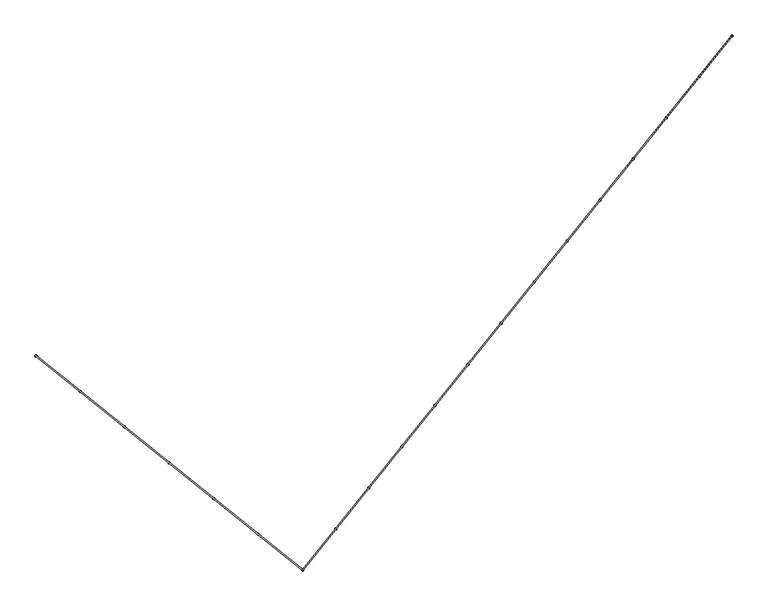
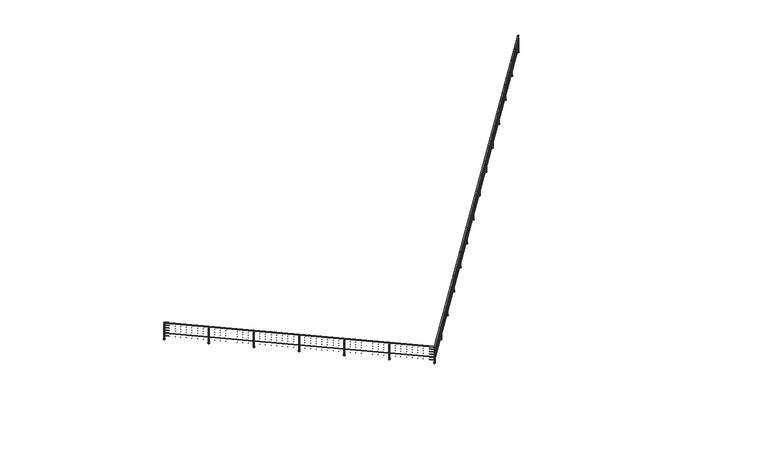
"""IFC4 building model written with IfcOpenShell, lengths in millimetres: railing geometry."""

from ifc_helpers import new_model, si_unit, point, frame, frame_2d, origin, place, context, project, spatial, circle_curve, ellipse_curve, trimmed, segment, composite_curve, outline, extrude, source, transform, mapped, element, save
from ifc_brep_helpers import plane_surface, cylinder_surface, advanced_brep


def railing_283a873e(model_context):
    return source(origin(), model_context, "Body", "SolidModel", [
        advanced_brep(
        [(16703.9390203, 14071.9773332, 12197.5), (16700.0406554, 14075.1082677, 12197.5), (-9274.6280116, 2130.9946489, 12197.5), (-9271.4970771, 2134.8930138, 12197.5), (687.6435705, -5870.1084734, 12197.5), (686.8761401, -5863.0791739, 12197.5)],
        [
            (0, 1, circle_curve(frame((16701.9898378, 14073.5428004, 12197.5), z_axis=(0.6261869005875139, 0.7796729862786083, 0.0), x_axis=(-0.7796729862786083, 0.6261869005875139, 0.0)), 2.5)),
            (1, 0, circle_curve(frame((16701.9898378, 14073.5428004, 12197.5), z_axis=(0.6261869005875139, 0.7796729862786083, 0.0), x_axis=(-0.7796729862786083, 0.6261869005875139, 0.0)), 2.5)),
            (2, 3, circle_curve(frame((-9273.0625444, 2132.9438313, 12197.5), z_axis=(-0.7796729862786094, 0.6261869005875127, 0.0), x_axis=(0.6261869005875127, 0.7796729862786094, 0.0)), 2.5)),
            (3, 2, circle_curve(frame((-9273.0625444, 2132.9438313, 12197.5), z_axis=(-0.7796729862786094, 0.6261869005875127, 0.0), x_axis=(0.6261869005875127, 0.7796729862786094, 0.0)), 2.5)),
            (0, 4),
            (4, 5, ellipse_curve(frame((687.2598553, -5866.5938237, 12197.5), z_axis=(0.9940930594011873, 0.1085310520099531, 0.0), x_axis=(-0.10853105200995282, 0.9940930594011875, 0.0)), 3.5355339, 2.5)),
            (5, 1),
            (5, 4, ellipse_curve(frame((687.2598553, -5866.5938237, 12197.5), z_axis=(0.9940930594011873, 0.1085310520099531, 0.0), x_axis=(-0.10853105200995282, 0.9940930594011875, 0.0)), 3.5355339, 2.5)),
            (4, 2),
            (3, 5),
        ],
        [
            plane_surface(frame((16701.9898378, 14073.5428004, 12200.0), z_axis=(0.6261869005875139, 0.7796729862786083, 0.0), x_axis=(0.7796729862786083, -0.6261869005875139, 0.0))),
            plane_surface(frame((-9273.0625444, 2132.9438313, 12200.0), z_axis=(-0.7796729862786096, 0.6261869005875125, 0.0), x_axis=(0.6261869005875125, 0.7796729862786096, 0.0))),
            cylinder_surface(frame((16701.9898378, 14073.5428004, 12197.5), z_axis=(0.6261869005875139, 0.7796729862786083, 0.0), x_axis=(-0.7796729862786083, 0.6261869005875139, 0.0)), 2.5),
            cylinder_surface(frame((687.2598553, -5866.5938237, 12197.5), z_axis=(0.7796729862786094, -0.6261869005875127, 0.0), x_axis=(0.6261869005875127, 0.7796729862786094, 0.0)), 2.5),
        ],
        [
            (0, [[1, 2]]),
            (1, [[3, 4]]),
            (2, [[-1, 5, 6, 7]]),
            (2, [[-2, -7, 8, -5]]),
            (3, [[-6, 9, -4, 10]]),
            (3, [[-8, -10, -3, -9]]),
        ],
    ),
        advanced_brep(
        [(16703.9390203, 14071.9773332, 12347.5), (16700.0406554, 14075.1082677, 12347.5), (-9274.6280116, 2130.9946489, 12347.5), (-9271.4970771, 2134.8930138, 12347.5), (687.6435705, -5870.1084734, 12347.5), (686.8761401, -5863.0791739, 12347.5)],
        [
            (0, 1, circle_curve(frame((16701.9898378, 14073.5428004, 12347.5), z_axis=(0.6261869005875139, 0.7796729862786083, 0.0), x_axis=(-0.7796729862786083, 0.6261869005875139, 0.0)), 2.5)),
            (1, 0, circle_curve(frame((16701.9898378, 14073.5428004, 12347.5), z_axis=(0.6261869005875139, 0.7796729862786083, 0.0), x_axis=(-0.7796729862786083, 0.6261869005875139, 0.0)), 2.5)),
            (2, 3, circle_curve(frame((-9273.0625444, 2132.9438313, 12347.5), z_axis=(-0.7796729862786094, 0.6261869005875127, 0.0), x_axis=(0.6261869005875127, 0.7796729862786094, 0.0)), 2.5)),
            (3, 2, circle_curve(frame((-9273.0625444, 2132.9438313, 12347.5), z_axis=(-0.7796729862786094, 0.6261869005875127, 0.0), x_axis=(0.6261869005875127, 0.7796729862786094, 0.0)), 2.5)),
            (0, 4),
            (4, 5, ellipse_curve(frame((687.2598553, -5866.5938237, 12347.5), z_axis=(0.9940930594011873, 0.1085310520099531, 0.0), x_axis=(-0.10853105200995282, 0.9940930594011875, 0.0)), 3.5355339, 2.5)),
            (5, 1),
            (5, 4, ellipse_curve(frame((687.2598553, -5866.5938237, 12347.5), z_axis=(0.9940930594011873, 0.1085310520099531, 0.0), x_axis=(-0.10853105200995282, 0.9940930594011875, 0.0)), 3.5355339, 2.5)),
            (4, 2),
            (3, 5),
        ],
        [
            plane_surface(frame((16701.9898378, 14073.5428004, 12350.0), z_axis=(0.6261869005875139, 0.7796729862786083, 0.0), x_axis=(0.7796729862786083, -0.6261869005875139, 0.0))),
            plane_surface(frame((-9273.0625444, 2132.9438313, 12350.0), z_axis=(-0.7796729862786096, 0.6261869005875125, 0.0), x_axis=(0.6261869005875125, 0.7796729862786096, 0.0))),
            cylinder_surface(frame((16701.9898378, 14073.5428004, 12347.5), z_axis=(0.6261869005875139, 0.7796729862786083, 0.0), x_axis=(-0.7796729862786083, 0.6261869005875139, 0.0)), 2.5),
            cylinder_surface(frame((687.2598553, -5866.5938237, 12347.5), z_axis=(0.7796729862786094, -0.6261869005875127, 0.0), x_axis=(0.6261869005875127, 0.7796729862786094, 0.0)), 2.5),
        ],
        [
            (0, [[1, 2]]),
            (1, [[3, 4]]),
            (2, [[-1, 5, 6, 7]]),
            (2, [[-2, -7, 8, -5]]),
            (3, [[-6, 9, -4, 10]]),
            (3, [[-8, -10, -3, -9]]),
        ],
    ),
        advanced_brep(
        [(16703.9390203, 14071.9773332, 12497.5), (16700.0406554, 14075.1082677, 12497.5), (-9274.6280116, 2130.9946489, 12497.5), (-9271.4970771, 2134.8930138, 12497.5), (687.6435705, -5870.1084734, 12497.5), (686.8761401, -5863.0791739, 12497.5)],
        [
            (0, 1, circle_curve(frame((16701.9898378, 14073.5428004, 12497.5), z_axis=(0.6261869005875139, 0.7796729862786083, 0.0), x_axis=(-0.7796729862786083, 0.6261869005875139, 0.0)), 2.5)),
            (1, 0, circle_curve(frame((16701.9898378, 14073.5428004, 12497.5), z_axis=(0.6261869005875139, 0.7796729862786083, 0.0), x_axis=(-0.7796729862786083, 0.6261869005875139, 0.0)), 2.5)),
            (2, 3, circle_curve(frame((-9273.0625444, 2132.9438313, 12497.5), z_axis=(-0.7796729862786094, 0.6261869005875127, 0.0), x_axis=(0.6261869005875127, 0.7796729862786094, 0.0)), 2.5)),
            (3, 2, circle_curve(frame((-9273.0625444, 2132.9438313, 12497.5), z_axis=(-0.7796729862786094, 0.6261869005875127, 0.0), x_axis=(0.6261869005875127, 0.7796729862786094, 0.0)), 2.5)),
            (0, 4),
            (4, 5, ellipse_curve(frame((687.2598553, -5866.5938237, 12497.5), z_axis=(0.9940930594011873, 0.1085310520099531, 0.0), x_axis=(-0.10853105200995282, 0.9940930594011875, 0.0)), 3.5355339, 2.5)),
            (5, 1),
            (5, 4, ellipse_curve(frame((687.2598553, -5866.5938237, 12497.5), z_axis=(0.9940930594011873, 0.1085310520099531, 0.0), x_axis=(-0.10853105200995282, 0.9940930594011875, 0.0)), 3.5355339, 2.5)),
            (4, 2),
            (3, 5),
        ],
        [
            plane_surface(frame((16701.9898378, 14073.5428004, 12500.0), z_axis=(0.6261869005875139, 0.7796729862786083, 0.0), x_axis=(0.7796729862786083, -0.6261869005875139, 0.0))),
            plane_surface(frame((-9273.0625444, 2132.9438313, 12500.0), z_axis=(-0.7796729862786096, 0.6261869005875125, 0.0), x_axis=(0.6261869005875125, 0.7796729862786096, 0.0))),
            cylinder_surface(frame((16701.9898378, 14073.5428004, 12497.5), z_axis=(0.6261869005875139, 0.7796729862786083, 0.0), x_axis=(-0.7796729862786083, 0.6261869005875139, 0.0)), 2.5),
            cylinder_surface(frame((687.2598553, -5866.5938237, 12497.5), z_axis=(0.7796729862786094, -0.6261869005875127, 0.0), x_axis=(0.6261869005875127, 0.7796729862786094, 0.0)), 2.5),
        ],
        [
            (0, [[1, 2]]),
            (1, [[3, 4]]),
            (2, [[-1, 5, 6, 7]]),
            (2, [[-2, -7, 8, -5]]),
            (3, [[-6, 9, -4, 10]]),
            (3, [[-8, -10, -3, -9]]),
        ],
    ),
        advanced_brep(
        [(16703.9390203, 14071.9773332, 12647.5), (16700.0406554, 14075.1082677, 12647.5), (687.6435705, -5870.1084734, 12647.5), (686.8761401, -5863.0791739, 12647.5), (-9274.6280116, 2130.9946489, 12647.5), (-9271.4970771, 2134.8930138, 12647.5)],
        [
            (0, 1, circle_curve(frame((16701.9898378, 14073.5428004, 12647.5), z_axis=(0.6261869005875139, 0.7796729862786083, 0.0), x_axis=(-0.7796729862786083, 0.6261869005875139, 0.0)), 2.5)),
            (1, 0, circle_curve(frame((16701.9898378, 14073.5428004, 12647.5), z_axis=(0.6261869005875139, 0.7796729862786083, 0.0), x_axis=(-0.7796729862786083, 0.6261869005875139, 0.0)), 2.5)),
            (0, 2),
            (2, 3, ellipse_curve(frame((687.2598553, -5866.5938237, 12647.5), z_axis=(0.9940930594011873, 0.1085310520099531, 0.0), x_axis=(-0.10853105200995282, 0.9940930594011875, 0.0)), 3.5355339, 2.5)),
            (3, 1),
            (3, 2, ellipse_curve(frame((687.2598553, -5866.5938237, 12647.5), z_axis=(0.9940930594011873, 0.1085310520099531, 0.0), x_axis=(-0.10853105200995282, 0.9940930594011875, 0.0)), 3.5355339, 2.5)),
            (4, 5, circle_curve(frame((-9273.0625444, 2132.9438313, 12647.5), z_axis=(-0.7796729862786094, 0.6261869005875127, 0.0), x_axis=(0.6261869005875127, 0.7796729862786094, 0.0)), 2.5)),
            (5, 4, circle_curve(frame((-9273.0625444, 2132.9438313, 12647.5), z_axis=(-0.7796729862786094, 0.6261869005875127, 0.0), x_axis=(0.6261869005875127, 0.7796729862786094, 0.0)), 2.5)),
            (2, 4),
            (5, 3),
        ],
        [
            plane_surface(frame((16701.9898378, 14073.5428004, 12650.0), z_axis=(0.6261869005875139, 0.7796729862786083, 0.0), x_axis=(0.7796729862786083, -0.6261869005875139, 0.0))),
            cylinder_surface(frame((16701.9898378, 14073.5428004, 12647.5), z_axis=(0.6261869005875139, 0.7796729862786083, 0.0), x_axis=(-0.7796729862786083, 0.6261869005875139, 0.0)), 2.5),
            plane_surface(frame((-9273.0625444, 2132.9438313, 12650.0), z_axis=(-0.7796729862786096, 0.6261869005875125, 0.0), x_axis=(0.6261869005875125, 0.7796729862786096, 0.0))),
            cylinder_surface(frame((687.2598553, -5866.5938237, 12647.5), z_axis=(0.7796729862786094, -0.6261869005875127, 0.0), x_axis=(0.6261869005875127, 0.7796729862786094, 0.0)), 2.5),
        ],
        [
            (0, [[1, 2]]),
            (1, [[-1, 3, 4, 5]]),
            (1, [[-2, -5, 6, -3]]),
            (2, [[7, 8]]),
            (3, [[-4, 9, -8, 10]]),
            (3, [[-6, -10, -7, -9]]),
        ],
    ),
        advanced_brep(
        [(16703.9390203, 14071.9773332, 12797.5), (16700.0406554, 14075.1082677, 12797.5), (687.6435705, -5870.1084734, 12797.5), (686.8761401, -5863.0791739, 12797.5), (-9274.6280116, 2130.9946489, 12797.5), (-9271.4970771, 2134.8930138, 12797.5)],
        [
            (0, 1, circle_curve(frame((16701.9898378, 14073.5428004, 12797.5), z_axis=(0.6261869005875139, 0.7796729862786083, 0.0), x_axis=(-0.7796729862786083, 0.6261869005875139, 0.0)), 2.5)),
            (1, 0, circle_curve(frame((16701.9898378, 14073.5428004, 12797.5), z_axis=(0.6261869005875139, 0.7796729862786083, 0.0), x_axis=(-0.7796729862786083, 0.6261869005875139, 0.0)), 2.5)),
            (0, 2),
            (2, 3, ellipse_curve(frame((687.2598553, -5866.5938237, 12797.5), z_axis=(0.9940930594011873, 0.1085310520099531, 0.0), x_axis=(-0.10853105200995282, 0.9940930594011875, 0.0)), 3.5355339, 2.5)),
            (3, 1),
            (3, 2, ellipse_curve(frame((687.2598553, -5866.5938237, 12797.5), z_axis=(0.9940930594011873, 0.1085310520099531, 0.0), x_axis=(-0.10853105200995282, 0.9940930594011875, 0.0)), 3.5355339, 2.5)),
            (4, 5, circle_curve(frame((-9273.0625444, 2132.9438313, 12797.5), z_axis=(-0.7796729862786094, 0.6261869005875127, 0.0), x_axis=(0.6261869005875127, 0.7796729862786094, 0.0)), 2.5)),
            (5, 4, circle_curve(frame((-9273.0625444, 2132.9438313, 12797.5), z_axis=(-0.7796729862786094, 0.6261869005875127, 0.0), x_axis=(0.6261869005875127, 0.7796729862786094, 0.0)), 2.5)),
            (2, 4),
            (5, 3),
        ],
        [
            plane_surface(frame((16701.9898378, 14073.5428004, 12800.0), z_axis=(0.6261869005875139, 0.7796729862786083, 0.0), x_axis=(0.7796729862786083, -0.6261869005875139, 0.0))),
            cylinder_surface(frame((16701.9898378, 14073.5428004, 12797.5), z_axis=(0.6261869005875139, 0.7796729862786083, 0.0), x_axis=(-0.7796729862786083, 0.6261869005875139, 0.0)), 2.5),
            plane_surface(frame((-9273.0625444, 2132.9438313, 12800.0), z_axis=(-0.7796729862786096, 0.6261869005875125, 0.0), x_axis=(0.6261869005875125, 0.7796729862786096, 0.0))),
            cylinder_surface(frame((687.2598553, -5866.5938237, 12797.5), z_axis=(0.7796729862786094, -0.6261869005875127, 0.0), x_axis=(0.6261869005875127, 0.7796729862786094, 0.0)), 2.5),
        ],
        [
            (0, [[1, 2]]),
            (1, [[-1, 3, 4, 5]]),
            (1, [[-2, -5, 6, -3]]),
            (2, [[7, 8]]),
            (3, [[-4, 9, -8, 10]]),
            (3, [[-6, -10, -7, -9]]),
        ],
    ),
        advanced_brep(
        [(16721.4816625, 14057.8881279, 12925.0), (16682.4980132, 14089.1974729, 12925.0), (691.0970075, -5901.7403208, 12925.0), (683.4227032, -5831.4473265, 12925.0), (-9288.7172169, 2113.4520067, 12925.0), (-9257.4078719, 2152.435656, 12925.0)],
        [
            (0, 1, circle_curve(frame((16701.9898378, 14073.5428004, 12925.0), z_axis=(0.6261869005875139, 0.7796729862786083, 0.0), x_axis=(-0.7796729862786083, 0.6261869005875139, 0.0)), 25.0)),
            (1, 0, circle_curve(frame((16701.9898378, 14073.5428004, 12925.0), z_axis=(0.6261869005875139, 0.7796729862786083, 0.0), x_axis=(-0.7796729862786083, 0.6261869005875139, 0.0)), 25.0)),
            (0, 2),
            (2, 3, ellipse_curve(frame((687.2598553, -5866.5938237, 12925.0), z_axis=(0.9940930594011873, 0.1085310520099531, 0.0), x_axis=(-0.10853105200995282, 0.9940930594011875, 0.0)), 35.3553391, 25.0)),
            (3, 1),
            (3, 2, ellipse_curve(frame((687.2598553, -5866.5938237, 12925.0), z_axis=(0.9940930594011873, 0.1085310520099531, 0.0), x_axis=(-0.10853105200995282, 0.9940930594011875, 0.0)), 35.3553391, 25.0)),
            (4, 5, circle_curve(frame((-9273.0625444, 2132.9438313, 12925.0), z_axis=(-0.7796729862786094, 0.6261869005875127, 0.0), x_axis=(0.6261869005875127, 0.7796729862786094, 0.0)), 25.0)),
            (5, 4, circle_curve(frame((-9273.0625444, 2132.9438313, 12925.0), z_axis=(-0.7796729862786094, 0.6261869005875127, 0.0), x_axis=(0.6261869005875127, 0.7796729862786094, 0.0)), 25.0)),
            (2, 4),
            (5, 3),
        ],
        [
            plane_surface(frame((16701.9898378, 14073.5428004, 12950.0), z_axis=(0.6261869005875139, 0.7796729862786083, 0.0), x_axis=(0.7796729862786083, -0.6261869005875139, 0.0))),
            cylinder_surface(frame((16701.9898378, 14073.5428004, 12925.0), z_axis=(0.6261869005875139, 0.7796729862786083, 0.0), x_axis=(-0.7796729862786083, 0.6261869005875139, 0.0)), 25.0),
            plane_surface(frame((-9273.0625444, 2132.9438313, 12950.0), z_axis=(-0.7796729862786096, 0.6261869005875125, 0.0), x_axis=(0.6261869005875125, 0.7796729862786096, 0.0))),
            cylinder_surface(frame((687.2598553, -5866.5938237, 12925.0), z_axis=(0.7796729862786094, -0.6261869005875127, 0.0), x_axis=(0.6261869005875127, 0.7796729862786094, 0.0)), 25.0),
        ],
        [
            (0, [[1, 2]]),
            (1, [[-1, 3, 4, 5]]),
            (1, [[-2, -5, 6, -3]]),
            (2, [[7, 8]]),
            (3, [[-4, 9, -8, 10]]),
            (3, [[-6, -10, -7, -9]]),
        ],
    ),
        extrude(outline(composite_curve([segment(trimmed(circle_curve(frame_2d((-7613.0088111, 799.6875555)), 5.0), [point((-7609.8778766, 803.5859204))], [point((-7616.1397456, 795.7891906))], False, "CARTESIAN"), True, "CONTINUOUS"), segment(trimmed(circle_curve(frame_2d((-7613.0088111, 799.6875555)), 5.0), [point((-7616.1397456, 795.7891906))], [point((-7609.8778766, 803.5859204))], False, "CARTESIAN"), True, "CONTINUOUS")], self_intersect=False)), frame((0.0, 0.0, 12825.0), z_axis=(0.0, 0.0, 1.0), x_axis=(1.0, 0.0, 0.0)), (0.0, 0.0, 1.0), 75.0),
        extrude(outline(composite_curve([segment(trimmed(circle_curve(frame_2d((-7613.0088111, 799.6875555)), 25.0), [point((-7597.3541386, 819.1793802))], [point((-7628.6634836, 780.1957309))], False, "CARTESIAN"), True, "CONTINUOUS"), segment(trimmed(circle_curve(frame_2d((-7613.0088111, 799.6875555)), 25.0), [point((-7628.6634836, 780.1957309))], [point((-7597.3541386, 819.1793802))], False, "CARTESIAN"), True, "CONTINUOUS")], self_intersect=False)), frame((0.0, 0.0, 12020.0), z_axis=(0.0, 0.0, 1.0), x_axis=(1.0, 0.0, 0.0)), (0.0, 0.0, 1.0), 805.0),
        extrude(outline(composite_curve([segment(trimmed(circle_curve(frame_2d((-7613.0088111, 799.6875555)), 40.0), [point((-7587.9613351, 830.874475))], [point((-7638.0562871, 768.5006361))], False, "CARTESIAN"), True, "CONTINUOUS"), segment(trimmed(circle_curve(frame_2d((-7613.0088111, 799.6875555)), 40.0), [point((-7638.0562871, 768.5006361))], [point((-7587.9613351, 830.874475))], False, "CARTESIAN"), True, "CONTINUOUS")], self_intersect=False)), frame((0.0, 0.0, 12000.0), z_axis=(0.0, 0.0, 1.0), x_axis=(1.0, 0.0, 0.0)), (0.0, 0.0, 1.0), 20.0),
        extrude(outline(composite_curve([segment(trimmed(circle_curve(frame_2d((-5952.9550778, -533.5687203)), 5.0), [point((-5949.8241433, -529.6703554))], [point((-5956.0860123, -537.4670853))], False, "CARTESIAN"), True, "CONTINUOUS"), segment(trimmed(circle_curve(frame_2d((-5952.9550778, -533.5687203)), 5.0), [point((-5956.0860123, -537.4670853))], [point((-5949.8241433, -529.6703554))], False, "CARTESIAN"), True, "CONTINUOUS")], self_intersect=False)), frame((0.0, 0.0, 12825.0), z_axis=(0.0, 0.0, 1.0), x_axis=(1.0, 0.0, 0.0)), (0.0, 0.0, 1.0), 75.0),
        extrude(outline(composite_curve([segment(trimmed(circle_curve(frame_2d((-5952.9550778, -533.5687203)), 25.0), [point((-5937.3004053, -514.0768957))], [point((-5968.6097503, -553.060545))], False, "CARTESIAN"), True, "CONTINUOUS"), segment(trimmed(circle_curve(frame_2d((-5952.9550778, -533.5687203)), 25.0), [point((-5968.6097503, -553.060545))], [point((-5937.3004053, -514.0768957))], False, "CARTESIAN"), True, "CONTINUOUS")], self_intersect=False)), frame((0.0, 0.0, 12020.0), z_axis=(0.0, 0.0, 1.0), x_axis=(1.0, 0.0, 0.0)), (0.0, 0.0, 1.0), 805.0),
        extrude(outline(composite_curve([segment(trimmed(circle_curve(frame_2d((-5952.9550778, -533.5687203)), 40.0), [point((-5927.9076018, -502.3818009))], [point((-5978.0025538, -564.7556398))], False, "CARTESIAN"), True, "CONTINUOUS"), segment(trimmed(circle_curve(frame_2d((-5952.9550778, -533.5687203)), 40.0), [point((-5978.0025538, -564.7556398))], [point((-5927.9076018, -502.3818009))], False, "CARTESIAN"), True, "CONTINUOUS")], self_intersect=False)), frame((0.0, 0.0, 12000.0), z_axis=(0.0, 0.0, 1.0), x_axis=(1.0, 0.0, 0.0)), (0.0, 0.0, 1.0), 20.0),
        extrude(outline(composite_curve([segment(trimmed(circle_curve(frame_2d((-4292.9013445, -1866.8249962)), 5.0), [point((-4289.77041, -1862.9266312))], [point((-4296.032279, -1870.7233611))], False, "CARTESIAN"), True, "CONTINUOUS"), segment(trimmed(circle_curve(frame_2d((-4292.9013445, -1866.8249962)), 5.0), [point((-4296.032279, -1870.7233611))], [point((-4289.77041, -1862.9266312))], False, "CARTESIAN"), True, "CONTINUOUS")], self_intersect=False)), frame((0.0, 0.0, 12825.0), z_axis=(0.0, 0.0, 1.0), x_axis=(1.0, 0.0, 0.0)), (0.0, 0.0, 1.0), 75.0),
        extrude(outline(composite_curve([segment(trimmed(circle_curve(frame_2d((-4292.9013445, -1866.8249962)), 25.0), [point((-4277.246672, -1847.3331715))], [point((-4308.5560171, -1886.3168208))], False, "CARTESIAN"), True, "CONTINUOUS"), segment(trimmed(circle_curve(frame_2d((-4292.9013445, -1866.8249962)), 25.0), [point((-4308.5560171, -1886.3168208))], [point((-4277.246672, -1847.3331715))], False, "CARTESIAN"), True, "CONTINUOUS")], self_intersect=False)), frame((0.0, 0.0, 12020.0), z_axis=(0.0, 0.0, 1.0), x_axis=(1.0, 0.0, 0.0)), (0.0, 0.0, 1.0), 805.0),
        extrude(outline(composite_curve([segment(trimmed(circle_curve(frame_2d((-4292.9013445, -1866.8249962)), 40.0), [point((-4267.8538685, -1835.6380767))], [point((-4317.9488206, -1898.0119156))], False, "CARTESIAN"), True, "CONTINUOUS"), segment(trimmed(circle_curve(frame_2d((-4292.9013445, -1866.8249962)), 40.0), [point((-4317.9488206, -1898.0119156))], [point((-4267.8538685, -1835.6380767))], False, "CARTESIAN"), True, "CONTINUOUS")], self_intersect=False)), frame((0.0, 0.0, 12000.0), z_axis=(0.0, 0.0, 1.0), x_axis=(1.0, 0.0, 0.0)), (0.0, 0.0, 1.0), 20.0),
        extrude(outline(composite_curve([segment(trimmed(circle_curve(frame_2d((-2632.8476113, -3200.081272)), 5.0), [point((-2629.7166768, -3196.1829071))], [point((-2635.9785458, -3203.9796369))], False, "CARTESIAN"), True, "CONTINUOUS"), segment(trimmed(circle_curve(frame_2d((-2632.8476113, -3200.081272)), 5.0), [point((-2635.9785458, -3203.9796369))], [point((-2629.7166768, -3196.1829071))], False, "CARTESIAN"), True, "CONTINUOUS")], self_intersect=False)), frame((0.0, 0.0, 12825.0), z_axis=(0.0, 0.0, 1.0), x_axis=(1.0, 0.0, 0.0)), (0.0, 0.0, 1.0), 75.0),
        extrude(outline(composite_curve([segment(trimmed(circle_curve(frame_2d((-2632.8476113, -3200.081272)), 25.0), [point((-2617.1929387, -3180.5894473))], [point((-2648.5022838, -3219.5730966))], False, "CARTESIAN"), True, "CONTINUOUS"), segment(trimmed(circle_curve(frame_2d((-2632.8476113, -3200.081272)), 25.0), [point((-2648.5022838, -3219.5730966))], [point((-2617.1929387, -3180.5894473))], False, "CARTESIAN"), True, "CONTINUOUS")], self_intersect=False)), frame((0.0, 0.0, 12020.0), z_axis=(0.0, 0.0, 1.0), x_axis=(1.0, 0.0, 0.0)), (0.0, 0.0, 1.0), 805.0),
        extrude(outline(composite_curve([segment(trimmed(circle_curve(frame_2d((-2632.8476113, -3200.081272)), 40.0), [point((-2607.8001352, -3168.8943525))], [point((-2657.8950873, -3231.2681914))], False, "CARTESIAN"), True, "CONTINUOUS"), segment(trimmed(circle_curve(frame_2d((-2632.8476113, -3200.081272)), 40.0), [point((-2657.8950873, -3231.2681914))], [point((-2607.8001352, -3168.8943525))], False, "CARTESIAN"), True, "CONTINUOUS")], self_intersect=False)), frame((0.0, 0.0, 12000.0), z_axis=(0.0, 0.0, 1.0), x_axis=(1.0, 0.0, 0.0)), (0.0, 0.0, 1.0), 20.0),
        extrude(outline(composite_curve([segment(trimmed(circle_curve(frame_2d((-972.793878, -4533.3375478)), 5.0), [point((-969.6629435, -4529.4391829))], [point((-975.9248125, -4537.2359128))], False, "CARTESIAN"), True, "CONTINUOUS"), segment(trimmed(circle_curve(frame_2d((-972.793878, -4533.3375478)), 5.0), [point((-975.9248125, -4537.2359128))], [point((-969.6629435, -4529.4391829))], False, "CARTESIAN"), True, "CONTINUOUS")], self_intersect=False)), frame((0.0, 0.0, 12825.0), z_axis=(0.0, 0.0, 1.0), x_axis=(1.0, 0.0, 0.0)), (0.0, 0.0, 1.0), 75.0),
        extrude(outline(composite_curve([segment(trimmed(circle_curve(frame_2d((-972.793878, -4533.3375478)), 25.0), [point((-957.1392055, -4513.8457232))], [point((-988.4485505, -4552.8293725))], False, "CARTESIAN"), True, "CONTINUOUS"), segment(trimmed(circle_curve(frame_2d((-972.793878, -4533.3375478)), 25.0), [point((-988.4485505, -4552.8293725))], [point((-957.1392055, -4513.8457232))], False, "CARTESIAN"), True, "CONTINUOUS")], self_intersect=False)), frame((0.0, 0.0, 12020.0), z_axis=(0.0, 0.0, 1.0), x_axis=(1.0, 0.0, 0.0)), (0.0, 0.0, 1.0), 805.0),
        extrude(outline(composite_curve([segment(trimmed(circle_curve(frame_2d((-972.793878, -4533.3375478)), 40.0), [point((-947.7464019, -4502.1506284))], [point((-997.841354, -4564.5244673))], False, "CARTESIAN"), True, "CONTINUOUS"), segment(trimmed(circle_curve(frame_2d((-972.793878, -4533.3375478)), 40.0), [point((-997.841354, -4564.5244673))], [point((-947.7464019, -4502.1506284))], False, "CARTESIAN"), True, "CONTINUOUS")], self_intersect=False)), frame((0.0, 0.0, 12000.0), z_axis=(0.0, 0.0, 1.0), x_axis=(1.0, 0.0, 0.0)), (0.0, 0.0, 1.0), 20.0),
        extrude(outline(composite_curve([segment(trimmed(circle_curve(frame_2d((687.2598553, -5866.5938237)), 5.0), [point((690.3907898, -5862.6954587))], [point((684.1289208, -5870.4921886))], False, "CARTESIAN"), True, "CONTINUOUS"), segment(trimmed(circle_curve(frame_2d((687.2598553, -5866.5938237)), 5.0), [point((684.1289208, -5870.4921886))], [point((690.3907898, -5862.6954587))], False, "CARTESIAN"), True, "CONTINUOUS")], self_intersect=False)), frame((0.0, 0.0, 12825.0), z_axis=(0.0, 0.0, 1.0), x_axis=(1.0, 0.0, 0.0)), (0.0, 0.0, 1.0), 75.0),
        extrude(outline(composite_curve([segment(trimmed(circle_curve(frame_2d((687.2598553, -5866.5938237)), 25.0), [point((702.9145278, -5847.101999))], [point((671.6051828, -5886.0856483))], False, "CARTESIAN"), True, "CONTINUOUS"), segment(trimmed(circle_curve(frame_2d((687.2598553, -5866.5938237)), 25.0), [point((671.6051828, -5886.0856483))], [point((702.9145278, -5847.101999))], False, "CARTESIAN"), True, "CONTINUOUS")], self_intersect=False)), frame((0.0, 0.0, 12020.0), z_axis=(0.0, 0.0, 1.0), x_axis=(1.0, 0.0, 0.0)), (0.0, 0.0, 1.0), 805.0),
        extrude(outline(composite_curve([segment(trimmed(circle_curve(frame_2d((687.2598553, -5866.5938237)), 40.0), [point((712.3073313, -5835.4069042))], [point((662.2123793, -5897.7807431))], False, "CARTESIAN"), True, "CONTINUOUS"), segment(trimmed(circle_curve(frame_2d((687.2598553, -5866.5938237)), 40.0), [point((662.2123793, -5897.7807431))], [point((712.3073313, -5835.4069042))], False, "CARTESIAN"), True, "CONTINUOUS")], self_intersect=False)), frame((0.0, 0.0, 12000.0), z_axis=(0.0, 0.0, 1.0), x_axis=(1.0, 0.0, 0.0)), (0.0, 0.0, 1.0), 20.0),
        extrude(outline(composite_curve([segment(trimmed(circle_curve(frame_2d((687.2598553, -5866.5938237)), 5.0), [point((683.3614904, -5863.4628892))], [point((691.1582202, -5869.7247582))], False, "CARTESIAN"), True, "CONTINUOUS"), segment(trimmed(circle_curve(frame_2d((687.2598553, -5866.5938237)), 5.0), [point((691.1582202, -5869.7247582))], [point((683.3614904, -5863.4628892))], False, "CARTESIAN"), True, "CONTINUOUS")], self_intersect=False)), frame((0.0, 0.0, 12825.0), z_axis=(0.0, 0.0, 1.0), x_axis=(1.0, 0.0, 0.0)), (0.0, 0.0, 1.0), 75.0),
        extrude(outline(composite_curve([segment(trimmed(circle_curve(frame_2d((687.2598553, -5866.5938237)), 25.0), [point((667.7680307, -5850.9391511))], [point((706.75168, -5882.2484962))], False, "CARTESIAN"), True, "CONTINUOUS"), segment(trimmed(circle_curve(frame_2d((687.2598553, -5866.5938237)), 25.0), [point((706.75168, -5882.2484962))], [point((667.7680307, -5850.9391511))], False, "CARTESIAN"), True, "CONTINUOUS")], self_intersect=False)), frame((0.0, 0.0, 12020.0), z_axis=(0.0, 0.0, 1.0), x_axis=(1.0, 0.0, 0.0)), (0.0, 0.0, 1.0), 805.0),
        extrude(outline(composite_curve([segment(trimmed(circle_curve(frame_2d((687.2598553, -5866.5938237)), 40.0), [point((656.0729359, -5841.5463476))], [point((718.4467748, -5891.6412997))], False, "CARTESIAN"), True, "CONTINUOUS"), segment(trimmed(circle_curve(frame_2d((687.2598553, -5866.5938237)), 40.0), [point((718.4467748, -5891.6412997))], [point((656.0729359, -5841.5463476))], False, "CARTESIAN"), True, "CONTINUOUS")], self_intersect=False)), frame((0.0, 0.0, 12000.0), z_axis=(0.0, 0.0, 1.0), x_axis=(1.0, 0.0, 0.0)), (0.0, 0.0, 1.0), 20.0),
        extrude(outline(composite_curve([segment(trimmed(circle_curve(frame_2d((1919.1621617, -4332.7371603)), 5.0), [point((1915.2637967, -4329.6062258))], [point((1923.0605266, -4335.8680948))], False, "CARTESIAN"), True, "CONTINUOUS"), segment(trimmed(circle_curve(frame_2d((1919.1621617, -4332.7371603)), 5.0), [point((1923.0605266, -4335.8680948))], [point((1915.2637967, -4329.6062258))], False, "CARTESIAN"), True, "CONTINUOUS")], self_intersect=False)), frame((0.0, 0.0, 12825.0), z_axis=(0.0, 0.0, 1.0), x_axis=(1.0, 0.0, 0.0)), (0.0, 0.0, 1.0), 75.0),
        extrude(outline(composite_curve([segment(trimmed(circle_curve(frame_2d((1919.1621617, -4332.7371603)), 25.0), [point((1899.670337, -4317.0824878))], [point((1938.6539863, -4348.3918328))], False, "CARTESIAN"), True, "CONTINUOUS"), segment(trimmed(circle_curve(frame_2d((1919.1621617, -4332.7371603)), 25.0), [point((1938.6539863, -4348.3918328))], [point((1899.670337, -4317.0824878))], False, "CARTESIAN"), True, "CONTINUOUS")], self_intersect=False)), frame((0.0, 0.0, 12020.0), z_axis=(0.0, 0.0, 1.0), x_axis=(1.0, 0.0, 0.0)), (0.0, 0.0, 1.0), 805.0),
        extrude(outline(composite_curve([segment(trimmed(circle_curve(frame_2d((1919.1621617, -4332.7371603)), 40.0), [point((1887.9752422, -4307.6896842))], [point((1950.3490811, -4357.7846363))], False, "CARTESIAN"), True, "CONTINUOUS"), segment(trimmed(circle_curve(frame_2d((1919.1621617, -4332.7371603)), 40.0), [point((1950.3490811, -4357.7846363))], [point((1887.9752422, -4307.6896842))], False, "CARTESIAN"), True, "CONTINUOUS")], self_intersect=False)), frame((0.0, 0.0, 12000.0), z_axis=(0.0, 0.0, 1.0), x_axis=(1.0, 0.0, 0.0)), (0.0, 0.0, 1.0), 20.0),
        extrude(outline(composite_curve([segment(trimmed(circle_curve(frame_2d((3151.064468, -2798.8804969)), 5.0), [point((3147.1661031, -2795.7495624))], [point((3154.9628329, -2802.0114314))], False, "CARTESIAN"), True, "CONTINUOUS"), segment(trimmed(circle_curve(frame_2d((3151.064468, -2798.8804969)), 5.0), [point((3154.9628329, -2802.0114314))], [point((3147.1661031, -2795.7495624))], False, "CARTESIAN"), True, "CONTINUOUS")], self_intersect=False)), frame((0.0, 0.0, 12825.0), z_axis=(0.0, 0.0, 1.0), x_axis=(1.0, 0.0, 0.0)), (0.0, 0.0, 1.0), 75.0),
        extrude(outline(composite_curve([segment(trimmed(circle_curve(frame_2d((3151.064468, -2798.8804969)), 25.0), [point((3131.5726434, -2783.2258244))], [point((3170.5562927, -2814.5351694))], False, "CARTESIAN"), True, "CONTINUOUS"), segment(trimmed(circle_curve(frame_2d((3151.064468, -2798.8804969)), 25.0), [point((3170.5562927, -2814.5351694))], [point((3131.5726434, -2783.2258244))], False, "CARTESIAN"), True, "CONTINUOUS")], self_intersect=False)), frame((0.0, 0.0, 12020.0), z_axis=(0.0, 0.0, 1.0), x_axis=(1.0, 0.0, 0.0)), (0.0, 0.0, 1.0), 805.0),
        extrude(outline(composite_curve([segment(trimmed(circle_curve(frame_2d((3151.064468, -2798.8804969)), 40.0), [point((3119.8775486, -2773.8330209))], [point((3182.2513875, -2823.9279729))], False, "CARTESIAN"), True, "CONTINUOUS"), segment(trimmed(circle_curve(frame_2d((3151.064468, -2798.8804969)), 40.0), [point((3182.2513875, -2823.9279729))], [point((3119.8775486, -2773.8330209))], False, "CARTESIAN"), True, "CONTINUOUS")], self_intersect=False)), frame((0.0, 0.0, 12000.0), z_axis=(0.0, 0.0, 1.0), x_axis=(1.0, 0.0, 0.0)), (0.0, 0.0, 1.0), 20.0),
        extrude(outline(composite_curve([segment(trimmed(circle_curve(frame_2d((4382.9667744, -1265.0238335)), 5.0), [point((4379.0684094, -1261.892899))], [point((4386.8651393, -1268.154768))], False, "CARTESIAN"), True, "CONTINUOUS"), segment(trimmed(circle_curve(frame_2d((4382.9667744, -1265.0238335)), 5.0), [point((4386.8651393, -1268.154768))], [point((4379.0684094, -1261.892899))], False, "CARTESIAN"), True, "CONTINUOUS")], self_intersect=False)), frame((0.0, 0.0, 12825.0), z_axis=(0.0, 0.0, 1.0), x_axis=(1.0, 0.0, 0.0)), (0.0, 0.0, 1.0), 75.0),
        extrude(outline(composite_curve([segment(trimmed(circle_curve(frame_2d((4382.9667744, -1265.0238335)), 25.0), [point((4363.4749497, -1249.369161))], [point((4402.458599, -1280.678506))], False, "CARTESIAN"), True, "CONTINUOUS"), segment(trimmed(circle_curve(frame_2d((4382.9667744, -1265.0238335)), 25.0), [point((4402.458599, -1280.678506))], [point((4363.4749497, -1249.369161))], False, "CARTESIAN"), True, "CONTINUOUS")], self_intersect=False)), frame((0.0, 0.0, 12020.0), z_axis=(0.0, 0.0, 1.0), x_axis=(1.0, 0.0, 0.0)), (0.0, 0.0, 1.0), 805.0),
        extrude(outline(composite_curve([segment(trimmed(circle_curve(frame_2d((4382.9667744, -1265.0238335)), 40.0), [point((4351.7798549, -1239.9763575))], [point((4414.1536938, -1290.0713095))], False, "CARTESIAN"), True, "CONTINUOUS"), segment(trimmed(circle_curve(frame_2d((4382.9667744, -1265.0238335)), 40.0), [point((4414.1536938, -1290.0713095))], [point((4351.7798549, -1239.9763575))], False, "CARTESIAN"), True, "CONTINUOUS")], self_intersect=False)), frame((0.0, 0.0, 12000.0), z_axis=(0.0, 0.0, 1.0), x_axis=(1.0, 0.0, 0.0)), (0.0, 0.0, 1.0), 20.0),
        extrude(outline(composite_curve([segment(trimmed(circle_curve(frame_2d((5614.8690807, 268.8328299)), 5.0), [point((5610.9707158, 271.9637644))], [point((5618.7674456, 265.7018954))], False, "CARTESIAN"), True, "CONTINUOUS"), segment(trimmed(circle_curve(frame_2d((5614.8690807, 268.8328299)), 5.0), [point((5618.7674456, 265.7018954))], [point((5610.9707158, 271.9637644))], False, "CARTESIAN"), True, "CONTINUOUS")], self_intersect=False)), frame((0.0, 0.0, 12825.0), z_axis=(0.0, 0.0, 1.0), x_axis=(1.0, 0.0, 0.0)), (0.0, 0.0, 1.0), 75.0),
        extrude(outline(composite_curve([segment(trimmed(circle_curve(frame_2d((5614.8690807, 268.8328299)), 25.0), [point((5595.377256, 284.4875024))], [point((5634.3609054, 253.1781574))], False, "CARTESIAN"), True, "CONTINUOUS"), segment(trimmed(circle_curve(frame_2d((5614.8690807, 268.8328299)), 25.0), [point((5634.3609054, 253.1781574))], [point((5595.377256, 284.4875024))], False, "CARTESIAN"), True, "CONTINUOUS")], self_intersect=False)), frame((0.0, 0.0, 12020.0), z_axis=(0.0, 0.0, 1.0), x_axis=(1.0, 0.0, 0.0)), (0.0, 0.0, 1.0), 805.0),
        extrude(outline(composite_curve([segment(trimmed(circle_curve(frame_2d((5614.8690807, 268.8328299)), 40.0), [point((5583.6821613, 293.8803059))], [point((5646.0560002, 243.7853539))], False, "CARTESIAN"), True, "CONTINUOUS"), segment(trimmed(circle_curve(frame_2d((5614.8690807, 268.8328299)), 40.0), [point((5646.0560002, 243.7853539))], [point((5583.6821613, 293.8803059))], False, "CARTESIAN"), True, "CONTINUOUS")], self_intersect=False)), frame((0.0, 0.0, 12000.0), z_axis=(0.0, 0.0, 1.0), x_axis=(1.0, 0.0, 0.0)), (0.0, 0.0, 1.0), 20.0),
        extrude(outline(composite_curve([segment(trimmed(circle_curve(frame_2d((6846.7713871, 1802.6894933)), 5.0), [point((6842.8730221, 1805.8204278))], [point((6850.669752, 1799.5585588))], False, "CARTESIAN"), True, "CONTINUOUS"), segment(trimmed(circle_curve(frame_2d((6846.7713871, 1802.6894933)), 5.0), [point((6850.669752, 1799.5585588))], [point((6842.8730221, 1805.8204278))], False, "CARTESIAN"), True, "CONTINUOUS")], self_intersect=False)), frame((0.0, 0.0, 12825.0), z_axis=(0.0, 0.0, 1.0), x_axis=(1.0, 0.0, 0.0)), (0.0, 0.0, 1.0), 75.0),
        extrude(outline(composite_curve([segment(trimmed(circle_curve(frame_2d((6846.7713871, 1802.6894933)), 25.0), [point((6827.2795624, 1818.3441658))], [point((6866.2632117, 1787.0348208))], False, "CARTESIAN"), True, "CONTINUOUS"), segment(trimmed(circle_curve(frame_2d((6846.7713871, 1802.6894933)), 25.0), [point((6866.2632117, 1787.0348208))], [point((6827.2795624, 1818.3441658))], False, "CARTESIAN"), True, "CONTINUOUS")], self_intersect=False)), frame((0.0, 0.0, 12020.0), z_axis=(0.0, 0.0, 1.0), x_axis=(1.0, 0.0, 0.0)), (0.0, 0.0, 1.0), 805.0),
        extrude(outline(composite_curve([segment(trimmed(circle_curve(frame_2d((6846.7713871, 1802.6894933)), 40.0), [point((6815.5844676, 1827.7369693))], [point((6877.9583065, 1777.6420173))], False, "CARTESIAN"), True, "CONTINUOUS"), segment(trimmed(circle_curve(frame_2d((6846.7713871, 1802.6894933)), 40.0), [point((6877.9583065, 1777.6420173))], [point((6815.5844676, 1827.7369693))], False, "CARTESIAN"), True, "CONTINUOUS")], self_intersect=False)), frame((0.0, 0.0, 12000.0), z_axis=(0.0, 0.0, 1.0), x_axis=(1.0, 0.0, 0.0)), (0.0, 0.0, 1.0), 20.0),
        extrude(outline(composite_curve([segment(trimmed(circle_curve(frame_2d((8078.6736934, 3336.5461567)), 5.0), [point((8074.7753285, 3339.6770912))], [point((8082.5720583, 3333.4152222))], False, "CARTESIAN"), True, "CONTINUOUS"), segment(trimmed(circle_curve(frame_2d((8078.6736934, 3336.5461567)), 5.0), [point((8082.5720583, 3333.4152222))], [point((8074.7753285, 3339.6770912))], False, "CARTESIAN"), True, "CONTINUOUS")], self_intersect=False)), frame((0.0, 0.0, 12825.0), z_axis=(0.0, 0.0, 1.0), x_axis=(1.0, 0.0, 0.0)), (0.0, 0.0, 1.0), 75.0),
        extrude(outline(composite_curve([segment(trimmed(circle_curve(frame_2d((8078.6736934, 3336.5461567)), 25.0), [point((8059.1818687, 3352.2008292))], [point((8098.1655181, 3320.8914842))], False, "CARTESIAN"), True, "CONTINUOUS"), segment(trimmed(circle_curve(frame_2d((8078.6736934, 3336.5461567)), 25.0), [point((8098.1655181, 3320.8914842))], [point((8059.1818687, 3352.2008292))], False, "CARTESIAN"), True, "CONTINUOUS")], self_intersect=False)), frame((0.0, 0.0, 12020.0), z_axis=(0.0, 0.0, 1.0), x_axis=(1.0, 0.0, 0.0)), (0.0, 0.0, 1.0), 805.0),
        extrude(outline(composite_curve([segment(trimmed(circle_curve(frame_2d((8078.6736934, 3336.5461567)), 40.0), [point((8047.486774, 3361.5936327))], [point((8109.8606129, 3311.4986807))], False, "CARTESIAN"), True, "CONTINUOUS"), segment(trimmed(circle_curve(frame_2d((8078.6736934, 3336.5461567)), 40.0), [point((8109.8606129, 3311.4986807))], [point((8047.486774, 3361.5936327))], False, "CARTESIAN"), True, "CONTINUOUS")], self_intersect=False)), frame((0.0, 0.0, 12000.0), z_axis=(0.0, 0.0, 1.0), x_axis=(1.0, 0.0, 0.0)), (0.0, 0.0, 1.0), 20.0),
        extrude(outline(composite_curve([segment(trimmed(circle_curve(frame_2d((9310.5759998, 4870.4028201)), 5.0), [point((9306.6776348, 4873.5337546))], [point((9314.4743647, 4867.2718856))], False, "CARTESIAN"), True, "CONTINUOUS"), segment(trimmed(circle_curve(frame_2d((9310.5759998, 4870.4028201)), 5.0), [point((9314.4743647, 4867.2718856))], [point((9306.6776348, 4873.5337546))], False, "CARTESIAN"), True, "CONTINUOUS")], self_intersect=False)), frame((0.0, 0.0, 12825.0), z_axis=(0.0, 0.0, 1.0), x_axis=(1.0, 0.0, 0.0)), (0.0, 0.0, 1.0), 75.0),
        extrude(outline(composite_curve([segment(trimmed(circle_curve(frame_2d((9310.5759998, 4870.4028201)), 25.0), [point((9291.0841751, 4886.0574926))], [point((9330.0678244, 4854.7481476))], False, "CARTESIAN"), True, "CONTINUOUS"), segment(trimmed(circle_curve(frame_2d((9310.5759998, 4870.4028201)), 25.0), [point((9330.0678244, 4854.7481476))], [point((9291.0841751, 4886.0574926))], False, "CARTESIAN"), True, "CONTINUOUS")], self_intersect=False)), frame((0.0, 0.0, 12020.0), z_axis=(0.0, 0.0, 1.0), x_axis=(1.0, 0.0, 0.0)), (0.0, 0.0, 1.0), 805.0),
        extrude(outline(composite_curve([segment(trimmed(circle_curve(frame_2d((9310.5759998, 4870.4028201)), 40.0), [point((9279.3890803, 4895.4502961))], [point((9341.7629192, 4845.3553441))], False, "CARTESIAN"), True, "CONTINUOUS"), segment(trimmed(circle_curve(frame_2d((9310.5759998, 4870.4028201)), 40.0), [point((9341.7629192, 4845.3553441))], [point((9279.3890803, 4895.4502961))], False, "CARTESIAN"), True, "CONTINUOUS")], self_intersect=False)), frame((0.0, 0.0, 12000.0), z_axis=(0.0, 0.0, 1.0), x_axis=(1.0, 0.0, 0.0)), (0.0, 0.0, 1.0), 20.0),
        extrude(outline(composite_curve([segment(trimmed(circle_curve(frame_2d((10542.4783061, 6404.2594835)), 5.0), [point((10538.5799412, 6407.390418))], [point((10546.376671, 6401.128549))], False, "CARTESIAN"), True, "CONTINUOUS"), segment(trimmed(circle_curve(frame_2d((10542.4783061, 6404.2594835)), 5.0), [point((10546.376671, 6401.128549))], [point((10538.5799412, 6407.390418))], False, "CARTESIAN"), True, "CONTINUOUS")], self_intersect=False)), frame((0.0, 0.0, 12825.0), z_axis=(0.0, 0.0, 1.0), x_axis=(1.0, 0.0, 0.0)), (0.0, 0.0, 1.0), 75.0),
        extrude(outline(composite_curve([segment(trimmed(circle_curve(frame_2d((10542.4783061, 6404.2594835)), 25.0), [point((10522.9864814, 6419.914156))], [point((10561.9701308, 6388.604811))], False, "CARTESIAN"), True, "CONTINUOUS"), segment(trimmed(circle_curve(frame_2d((10542.4783061, 6404.2594835)), 25.0), [point((10561.9701308, 6388.604811))], [point((10522.9864814, 6419.914156))], False, "CARTESIAN"), True, "CONTINUOUS")], self_intersect=False)), frame((0.0, 0.0, 12020.0), z_axis=(0.0, 0.0, 1.0), x_axis=(1.0, 0.0, 0.0)), (0.0, 0.0, 1.0), 805.0),
        extrude(outline(composite_curve([segment(trimmed(circle_curve(frame_2d((10542.4783061, 6404.2594835)), 40.0), [point((10511.2913866, 6429.3069595))], [point((10573.6652256, 6379.2120074))], False, "CARTESIAN"), True, "CONTINUOUS"), segment(trimmed(circle_curve(frame_2d((10542.4783061, 6404.2594835)), 40.0), [point((10573.6652256, 6379.2120074))], [point((10511.2913866, 6429.3069595))], False, "CARTESIAN"), True, "CONTINUOUS")], self_intersect=False)), frame((0.0, 0.0, 12000.0), z_axis=(0.0, 0.0, 1.0), x_axis=(1.0, 0.0, 0.0)), (0.0, 0.0, 1.0), 20.0),
        extrude(outline(composite_curve([segment(trimmed(circle_curve(frame_2d((11774.3806124, 7938.1161469)), 5.0), [point((11770.4822475, 7941.2470814))], [point((11778.2789774, 7934.9852124))], False, "CARTESIAN"), True, "CONTINUOUS"), segment(trimmed(circle_curve(frame_2d((11774.3806124, 7938.1161469)), 5.0), [point((11778.2789774, 7934.9852124))], [point((11770.4822475, 7941.2470814))], False, "CARTESIAN"), True, "CONTINUOUS")], self_intersect=False)), frame((0.0, 0.0, 12825.0), z_axis=(0.0, 0.0, 1.0), x_axis=(1.0, 0.0, 0.0)), (0.0, 0.0, 1.0), 75.0),
        extrude(outline(composite_curve([segment(trimmed(circle_curve(frame_2d((11774.3806124, 7938.1161469)), 25.0), [point((11754.8887878, 7953.7708194))], [point((11793.8724371, 7922.4614743))], False, "CARTESIAN"), True, "CONTINUOUS"), segment(trimmed(circle_curve(frame_2d((11774.3806124, 7938.1161469)), 25.0), [point((11793.8724371, 7922.4614743))], [point((11754.8887878, 7953.7708194))], False, "CARTESIAN"), True, "CONTINUOUS")], self_intersect=False)), frame((0.0, 0.0, 12020.0), z_axis=(0.0, 0.0, 1.0), x_axis=(1.0, 0.0, 0.0)), (0.0, 0.0, 1.0), 805.0),
        extrude(outline(composite_curve([segment(trimmed(circle_curve(frame_2d((11774.3806124, 7938.1161469)), 40.0), [point((11743.193693, 7963.1636229))], [point((11805.5675319, 7913.0686708))], False, "CARTESIAN"), True, "CONTINUOUS"), segment(trimmed(circle_curve(frame_2d((11774.3806124, 7938.1161469)), 40.0), [point((11805.5675319, 7913.0686708))], [point((11743.193693, 7963.1636229))], False, "CARTESIAN"), True, "CONTINUOUS")], self_intersect=False)), frame((0.0, 0.0, 12000.0), z_axis=(0.0, 0.0, 1.0), x_axis=(1.0, 0.0, 0.0)), (0.0, 0.0, 1.0), 20.0),
        extrude(outline(composite_curve([segment(trimmed(circle_curve(frame_2d((13006.2829188, 9471.9728102)), 5.0), [point((13002.3845539, 9475.1037447))], [point((13010.1812837, 9468.8418757))], False, "CARTESIAN"), True, "CONTINUOUS"), segment(trimmed(circle_curve(frame_2d((13006.2829188, 9471.9728102)), 5.0), [point((13010.1812837, 9468.8418757))], [point((13002.3845539, 9475.1037447))], False, "CARTESIAN"), True, "CONTINUOUS")], self_intersect=False)), frame((0.0, 0.0, 12825.0), z_axis=(0.0, 0.0, 1.0), x_axis=(1.0, 0.0, 0.0)), (0.0, 0.0, 1.0), 75.0),
        extrude(outline(composite_curve([segment(trimmed(circle_curve(frame_2d((13006.2829188, 9471.9728102)), 25.0), [point((12986.7910941, 9487.6274828))], [point((13025.7747435, 9456.3181377))], False, "CARTESIAN"), True, "CONTINUOUS"), segment(trimmed(circle_curve(frame_2d((13006.2829188, 9471.9728102)), 25.0), [point((13025.7747435, 9456.3181377))], [point((12986.7910941, 9487.6274828))], False, "CARTESIAN"), True, "CONTINUOUS")], self_intersect=False)), frame((0.0, 0.0, 12020.0), z_axis=(0.0, 0.0, 1.0), x_axis=(1.0, 0.0, 0.0)), (0.0, 0.0, 1.0), 805.0),
        extrude(outline(composite_curve([segment(trimmed(circle_curve(frame_2d((13006.2829188, 9471.9728102)), 40.0), [point((12975.0959993, 9497.0202863))], [point((13037.4698382, 9446.9253342))], False, "CARTESIAN"), True, "CONTINUOUS"), segment(trimmed(circle_curve(frame_2d((13006.2829188, 9471.9728102)), 40.0), [point((13037.4698382, 9446.9253342))], [point((12975.0959993, 9497.0202863))], False, "CARTESIAN"), True, "CONTINUOUS")], self_intersect=False)), frame((0.0, 0.0, 12000.0), z_axis=(0.0, 0.0, 1.0), x_axis=(1.0, 0.0, 0.0)), (0.0, 0.0, 1.0), 20.0),
        extrude(outline(composite_curve([segment(trimmed(circle_curve(frame_2d((14238.1852251, 11005.8294736)), 5.0), [point((14234.2868602, 11008.9604081))], [point((14242.0835901, 11002.6985391))], False, "CARTESIAN"), True, "CONTINUOUS"), segment(trimmed(circle_curve(frame_2d((14238.1852251, 11005.8294736)), 5.0), [point((14242.0835901, 11002.6985391))], [point((14234.2868602, 11008.9604081))], False, "CARTESIAN"), True, "CONTINUOUS")], self_intersect=False)), frame((0.0, 0.0, 12825.0), z_axis=(0.0, 0.0, 1.0), x_axis=(1.0, 0.0, 0.0)), (0.0, 0.0, 1.0), 75.0),
        extrude(outline(composite_curve([segment(trimmed(circle_curve(frame_2d((14238.1852251, 11005.8294736)), 25.0), [point((14218.6934005, 11021.4841462))], [point((14257.6770498, 10990.1748011))], False, "CARTESIAN"), True, "CONTINUOUS"), segment(trimmed(circle_curve(frame_2d((14238.1852251, 11005.8294736)), 25.0), [point((14257.6770498, 10990.1748011))], [point((14218.6934005, 11021.4841462))], False, "CARTESIAN"), True, "CONTINUOUS")], self_intersect=False)), frame((0.0, 0.0, 12020.0), z_axis=(0.0, 0.0, 1.0), x_axis=(1.0, 0.0, 0.0)), (0.0, 0.0, 1.0), 805.0),
        extrude(outline(composite_curve([segment(trimmed(circle_curve(frame_2d((14238.1852251, 11005.8294736)), 40.0), [point((14206.9983057, 11030.8769497))], [point((14269.3721446, 10980.7819976))], False, "CARTESIAN"), True, "CONTINUOUS"), segment(trimmed(circle_curve(frame_2d((14238.1852251, 11005.8294736)), 40.0), [point((14269.3721446, 10980.7819976))], [point((14206.9983057, 11030.8769497))], False, "CARTESIAN"), True, "CONTINUOUS")], self_intersect=False)), frame((0.0, 0.0, 12000.0), z_axis=(0.0, 0.0, 1.0), x_axis=(1.0, 0.0, 0.0)), (0.0, 0.0, 1.0), 20.0),
        extrude(outline(composite_curve([segment(trimmed(circle_curve(frame_2d((15470.0875315, 12539.686137)), 5.0), [point((15466.1891666, 12542.8170715))], [point((15473.9858964, 12536.5552025))], False, "CARTESIAN"), True, "CONTINUOUS"), segment(trimmed(circle_curve(frame_2d((15470.0875315, 12539.686137)), 5.0), [point((15473.9858964, 12536.5552025))], [point((15466.1891666, 12542.8170715))], False, "CARTESIAN"), True, "CONTINUOUS")], self_intersect=False)), frame((0.0, 0.0, 12825.0), z_axis=(0.0, 0.0, 1.0), x_axis=(1.0, 0.0, 0.0)), (0.0, 0.0, 1.0), 75.0),
        extrude(outline(composite_curve([segment(trimmed(circle_curve(frame_2d((15470.0875315, 12539.686137)), 25.0), [point((15450.5957068, 12555.3408095))], [point((15489.5793561, 12524.0314645))], False, "CARTESIAN"), True, "CONTINUOUS"), segment(trimmed(circle_curve(frame_2d((15470.0875315, 12539.686137)), 25.0), [point((15489.5793561, 12524.0314645))], [point((15450.5957068, 12555.3408095))], False, "CARTESIAN"), True, "CONTINUOUS")], self_intersect=False)), frame((0.0, 0.0, 12020.0), z_axis=(0.0, 0.0, 1.0), x_axis=(1.0, 0.0, 0.0)), (0.0, 0.0, 1.0), 805.0),
        extrude(outline(composite_curve([segment(trimmed(circle_curve(frame_2d((15470.0875315, 12539.686137)), 40.0), [point((15438.900612, 12564.7336131))], [point((15501.2744509, 12514.638661))], False, "CARTESIAN"), True, "CONTINUOUS"), segment(trimmed(circle_curve(frame_2d((15470.0875315, 12539.686137)), 40.0), [point((15501.2744509, 12514.638661))], [point((15438.900612, 12564.7336131))], False, "CARTESIAN"), True, "CONTINUOUS")], self_intersect=False)), frame((0.0, 0.0, 12000.0), z_axis=(0.0, 0.0, 1.0), x_axis=(1.0, 0.0, 0.0)), (0.0, 0.0, 1.0), 20.0),
        extrude(outline(composite_curve([segment(trimmed(circle_curve(frame_2d((-9253.5707197, 2117.2891588)), 5.0), [point((-9250.4397852, 2121.1875238))], [point((-9256.7016542, 2113.3907939))], False, "CARTESIAN"), True, "CONTINUOUS"), segment(trimmed(circle_curve(frame_2d((-9253.5707197, 2117.2891588)), 5.0), [point((-9256.7016542, 2113.3907939))], [point((-9250.4397852, 2121.1875238))], False, "CARTESIAN"), True, "CONTINUOUS")], self_intersect=False)), frame((0.0, 0.0, 12825.0), z_axis=(0.0, 0.0, 1.0), x_axis=(1.0, 0.0, 0.0)), (0.0, 0.0, 1.0), 75.0),
        extrude(outline(composite_curve([segment(trimmed(circle_curve(frame_2d((-9253.5707197, 2117.2891588)), 25.0), [point((-9237.9160472, 2136.7809835))], [point((-9269.2253923, 2097.7973342))], False, "CARTESIAN"), True, "CONTINUOUS"), segment(trimmed(circle_curve(frame_2d((-9253.5707197, 2117.2891588)), 25.0), [point((-9269.2253923, 2097.7973342))], [point((-9237.9160472, 2136.7809835))], False, "CARTESIAN"), True, "CONTINUOUS")], self_intersect=False)), frame((0.0, 0.0, 12020.0), z_axis=(0.0, 0.0, 1.0), x_axis=(1.0, 0.0, 0.0)), (0.0, 0.0, 1.0), 805.0),
        extrude(outline(composite_curve([segment(trimmed(circle_curve(frame_2d((-9253.5707197, 2117.2891588)), 40.0), [point((-9228.5232437, 2148.4760783))], [point((-9278.6181958, 2086.1022394))], False, "CARTESIAN"), True, "CONTINUOUS"), segment(trimmed(circle_curve(frame_2d((-9253.5707197, 2117.2891588)), 40.0), [point((-9278.6181958, 2086.1022394))], [point((-9228.5232437, 2148.4760783))], False, "CARTESIAN"), True, "CONTINUOUS")], self_intersect=False)), frame((0.0, 0.0, 12000.0), z_axis=(0.0, 0.0, 1.0), x_axis=(1.0, 0.0, 0.0)), (0.0, 0.0, 1.0), 20.0),
        extrude(outline(composite_curve([segment(trimmed(circle_curve(frame_2d((16686.3351653, 14054.0509758)), 5.0), [point((16682.4368004, 14057.1819103))], [point((16690.2335303, 14050.9200413))], False, "CARTESIAN"), True, "CONTINUOUS"), segment(trimmed(circle_curve(frame_2d((16686.3351653, 14054.0509758)), 5.0), [point((16690.2335303, 14050.9200413))], [point((16682.4368004, 14057.1819103))], False, "CARTESIAN"), True, "CONTINUOUS")], self_intersect=False)), frame((0.0, 0.0, 12825.0), z_axis=(0.0, 0.0, 1.0), x_axis=(1.0, 0.0, 0.0)), (0.0, 0.0, 1.0), 75.0),
        extrude(outline(composite_curve([segment(trimmed(circle_curve(frame_2d((16686.3351653, 14054.0509758)), 25.0), [point((16666.8433407, 14069.7056483))], [point((16705.82699, 14038.3963032))], False, "CARTESIAN"), True, "CONTINUOUS"), segment(trimmed(circle_curve(frame_2d((16686.3351653, 14054.0509758)), 25.0), [point((16705.82699, 14038.3963032))], [point((16666.8433407, 14069.7056483))], False, "CARTESIAN"), True, "CONTINUOUS")], self_intersect=False)), frame((0.0, 0.0, 12020.0), z_axis=(0.0, 0.0, 1.0), x_axis=(1.0, 0.0, 0.0)), (0.0, 0.0, 1.0), 805.0),
        extrude(outline(composite_curve([segment(trimmed(circle_curve(frame_2d((16686.3351653, 14054.0509758)), 40.0), [point((16655.1482459, 14079.0984518))], [point((16717.5220848, 14029.0034997))], False, "CARTESIAN"), True, "CONTINUOUS"), segment(trimmed(circle_curve(frame_2d((16686.3351653, 14054.0509758)), 40.0), [point((16717.5220848, 14029.0034997))], [point((16655.1482459, 14079.0984518))], False, "CARTESIAN"), True, "CONTINUOUS")], self_intersect=False)), frame((0.0, 0.0, 12000.0), z_axis=(0.0, 0.0, 1.0), x_axis=(1.0, 0.0, 0.0)), (0.0, 0.0, 1.0), 20.0),
    ])


if __name__ == "__main__":
    model = new_model("IFC4")
    model_context = context("Model", 3, world=origin())
    ifc_project = project(units=[si_unit("LENGTHUNIT", "METRE", prefix="MILLI")], contexts=[model_context])
    site = spatial("IfcSite", under=ifc_project)
    building = spatial("IfcBuilding", under=site)
    placement = place(None, origin())
    railing_shape = railing_283a873e(model_context)
    element("IfcRailing", 1, at=placement, inside=building, context=model_context, shape_type="MappedRepresentation", body=[
        mapped(railing_shape, transform((0.0, 0.0, 0.0), x_axis=(1.0, 0.0, 0.0), y_axis=(0.0, 1.0, 0.0), z_axis=(0.0, 0.0, 1.0))),
    ])
    save(model, "model.ifc")

# Revit data of these elements
# Element 1 (IfcRailing)
#   Materials on its faces: ".aço inox_growarq", ".alumínio preto_growarq"
# Materials
#   ".aço inox_growarq": class "Metal", colour RGB 200 200 200, transparency 0, Description = "aço inoxidável polido", Cost = 0
#   ".alumínio preto_growarq": class "Metal", colour RGB 30 30 30, transparency 0.01, Comments = ".Enviar detalhamento das esquadrias para ter orçamento preciso", Description = "Alumínio acetinado preto", Cost = 0
